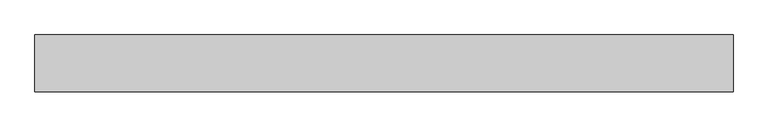
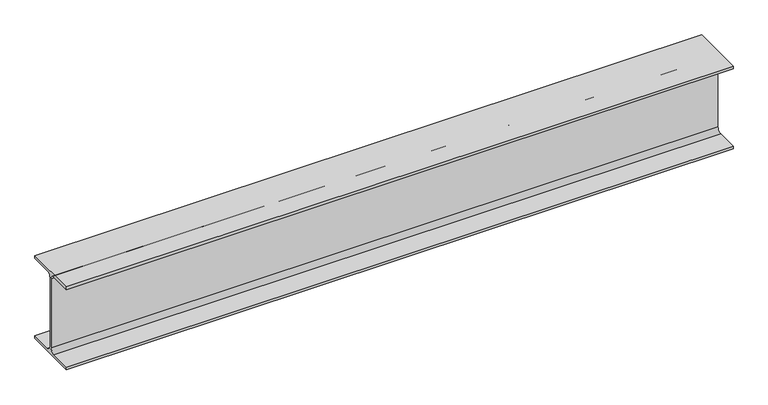
"""IFC4 building model written with IfcOpenShell, lengths in millimetres: beam geometry, 0912_Steel Framing_H-KSD3502 : H_SB_ASB_H-482x300x11x15."""

from ifc_helpers import new_model, si_unit, point, frame, frame_2d, origin, place, context, project, spatial, polyline, circle_curve, trimmed, segment, composite_curve, outline, extrude, source, transform, mapped, element, save


def beam_68d1f70f(model_context):
    return source(origin(), model_context, "Body", "SweptSolid", [
        extrude(outline(composite_curve([segment(polyline([(150.0, -226.0), (150.0, -241.0), (-150.0, -241.0), (-150.0, -226.0), (-31.5, -226.0)]), True, "CONTINUOUS"), segment(trimmed(circle_curve(frame_2d((-31.5, -200.0)), 26.0), [point((-31.5, -226.0))], [point((-5.5, -200.0))], True, "CARTESIAN"), True, "CONTINUOUS"), segment(polyline([(-5.5, -200.0), (-5.5, 200.0)]), True, "CONTINUOUS"), segment(trimmed(circle_curve(frame_2d((-31.5, 200.0)), 26.0), [point((-5.5, 200.0))], [point((-31.5, 226.0))], True, "CARTESIAN"), True, "CONTINUOUS"), segment(polyline([(-31.5, 226.0), (-150.0, 226.0), (-150.0, 241.0), (150.0, 241.0), (150.0, 226.0), (31.5, 226.0)]), True, "CONTINUOUS"), segment(trimmed(circle_curve(frame_2d((31.5, 200.0)), 26.0), [point((31.5, 226.0))], [point((5.5, 200.0))], True, "CARTESIAN"), True, "CONTINUOUS"), segment(polyline([(5.5, 200.0), (5.5, -200.0)]), True, "CONTINUOUS"), segment(trimmed(circle_curve(frame_2d((31.5, -200.0)), 26.0), [point((5.5, -200.0))], [point((31.5, -226.0))], True, "CARTESIAN"), True, "CONTINUOUS"), segment(polyline([(31.5, -226.0), (150.0, -226.0)]), True, "CONTINUOUS")], self_intersect=False)), frame((-1837.3, 0.0, 0.0), z_axis=(1.0, 0.0, 0.0), x_axis=(0.0, 1.0, 0.0)), (0.0, 0.0, 1.0), 3674.6),
    ])


if __name__ == "__main__":
    model = new_model("IFC4")
    model_context = context("Model", 3, world=origin())
    ifc_project = project(units=[si_unit("LENGTHUNIT", "METRE", prefix="MILLI")], contexts=[model_context])
    site = spatial("IfcSite", under=ifc_project)
    building = spatial("IfcBuilding", under=site)
    placement = place(None, origin())
    beam_shape = beam_68d1f70f(model_context)
    element("IfcBeam", 1, ObjectType="0912_Steel Framing_H-KSD3502 : H_SB_ASB_H-482x300x11x15", at=placement, inside=building, context=model_context, shape_type="MappedRepresentation", body=[
        mapped(beam_shape, transform((0.0, 0.0, 0.0), x_axis=(1.0, 0.0, 0.0), y_axis=(0.0, 1.0, 0.0), z_axis=(0.0, 0.0, 1.0))),
    ])
    save(model, "model.ifc")

# Revit data of these elements
# Type "0912_Steel Framing_H-KSD3502 : H_SB_ASB_H-482x300x11x15"
#   H_WM Code_1 = "S01AA001-00001 | Main Steel Structure Fabrication Work | Shelter/Building | Heavy Steel - Standard (Weight≥90KG/M) | Material: (   )"
#   H_WM Code_2 = "S03AA027-00001 | Main Steel Structure Erection Work | Shelter/Building | Heavy Steel (Weight≥90KG/M) | Material: (   )"
#   H_WM Code_3 = "S01AA010-00001 | Main Steel Structure Fabrication Work | Shelter/Building | Steel Painting/Coating | for Non-Fireproofed Steel Surface, Surface Preparation, Primer, Second & Final Coat | Material: (   )"
#   H_Q'ty Cal Type Tag = "SB-Q2"
#   Width = 30.0 cm
#   Web Thickness = 1.1 cm
#   Web Fillet = 2.6 cm
#   Warping Constant = 3680000.0 cm⁶
#   W = 0
#   Torsional Moment of Inertia = 88.2192 cm⁴
#   Section Area = 145.5 cm²
#   Plastic Modulus weak axis = 695.0 cm³
#   Plastic Modulus strong axis = 2790.0 cm³
#   Perimeter = 2.10 m²/m
#   Nominal Weight = 114.00 kgf/m
#   Moment of Inertia weak axis = 6760.00 cm⁴
#   Moment of Inertia strong axis = 60400.00 cm⁴
#   Height = 48.2 cm
#   Flange Thickness = 1.5 cm
#   Elastic Modulus weak axis = 451.0 cm³
#   Elastic Modulus strong axis = 2500.0 cm³
#   Centroid Vertical = 24.1 cm
#   Centroid Horizontal = 15.0 cm
#   Ix = 604000000
#   Length [instance default] = 1.5240 m
#   Zx = 2790000
#   b = 0.3000 m
#   h = 0.4820 m
#   r = 0.0260 m
#   s = 0.0110 m
#   t = 0.0150 m
#   A = 0.01455 m²
#   Structural Material [instance default] = Steel, 45-345
#   Assembly Code = ""
# Element 1 (IfcBeam, "0912_Steel Framing_H-KSD3502 : H_SB_ASB_H-482x300x11x15")
#   Structural Material = none
# Materials
#   "Steel, 45-345": class "Metal", colour RGB 189 187 185, transparency 0, Description = "Steel 345 MPa", Cost = 0
